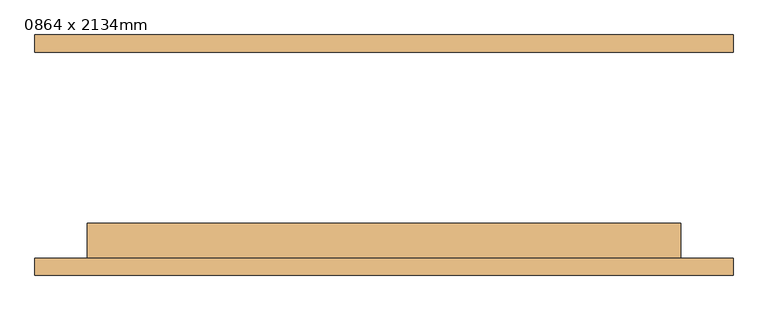
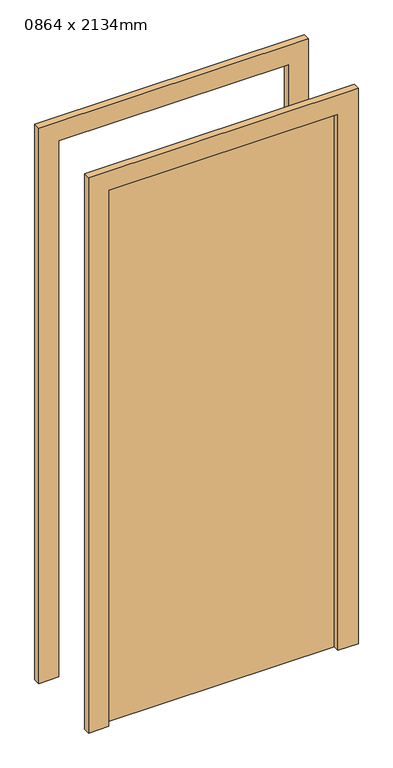
"""IFC4 building model written with IfcOpenShell, lengths in millimetres: door geometry, M_Folha única : 0864 x 2134mm."""

from ifc_helpers import new_model, si_unit, frame, origin, origin_with_axes, place, context, project, spatial, polyline, outline, extrude, source, transform, mapped, element, save


def door_0864_x_2134mm_1beed8f0(model_context):
    return source(origin(), model_context, "Body", "SweptSolid", [
        extrude(outline(polyline([(2210.0, -508.0), (0.0, -508.0), (0.0, -432.0), (2134.0, -432.0), (2134.0, 432.0), (0.0, 432.0), (0.0, 508.0), (2210.0, 508.0), (2210.0, -508.0)])), frame((0.0, -175.0, 0.0), z_axis=(0.0, 1.0, 0.0), x_axis=(0.0, 0.0, 1.0)), (0.0, 0.0, 1.0), 25.0),
        extrude(outline(polyline([(2210.0, 508.0), (2210.0, -508.0), (0.0, -508.0), (0.0, -432.0), (2134.0, -432.0), (2134.0, 432.0), (0.0, 432.0), (0.0, 508.0), (2210.0, 508.0)])), frame((0.0, 150.0, 0.0), z_axis=(0.0, 1.0, 0.0), x_axis=(0.0, 0.0, 1.0)), (0.0, 0.0, 1.0), 25.0),
        extrude(outline(polyline([(432.0, -99.0), (432.0, -150.0), (-432.0, -150.0), (-432.0, -99.0), (432.0, -99.0)])), origin_with_axes(), (0.0, 0.0, 1.0), 2134.0),
    ])


if __name__ == "__main__":
    model = new_model("IFC4")
    model_context = context("Model", 3, world=origin())
    ifc_project = project(units=[si_unit("LENGTHUNIT", "METRE", prefix="MILLI")], contexts=[model_context])
    site = spatial("IfcSite", under=ifc_project)
    building = spatial("IfcBuilding", under=site)
    placement = place(None, origin())
    door_0864_x_2134mm_shape = door_0864_x_2134mm_1beed8f0(model_context)
    element("IfcDoor", 1, ObjectType="M_Folha única : 0864 x 2134mm", at=placement, inside=building, context=model_context, shape_type="MappedRepresentation", body=[
        mapped(door_0864_x_2134mm_shape, transform((0.0, 0.0, 0.0), x_axis=(1.0, 0.0, 0.0), y_axis=(0.0, 1.0, 0.0), z_axis=(0.0, 0.0, 1.0))),
    ])
    save(model, "model.ifc")

# Revit data of these elements
# Project information
#   Opção de desenho = "Modelo principal"
#   Data de emissão do projeto = "Data de emissão"
#   Status do projeto = "Status do projeto"
#   Nome do cliente = "Proprietário"
#   Endereço do projeto = "Insira aqui o endereço"
#   Nome do projeto = "Nome do projeto"
#   Número do projeto = "0001"
# Type "M_Folha única : 0864 x 2134mm"
#   Type Mark = "22"
#   Construction Type Id = "MDOOR"
#   Analytic Construction = "Metal"
#   Thickness = 0.051 m
#   Thermal Resistance (R) = 0.270117 (m²·K)/W
#   Heat Transfer Coefficient (U) = 3.7021 W/(m²·K)
#   Height = 2.134 m
#   Projeção da apara externa = 0.025 m
#   Projeção da apara interna = 0.025 m
#   Largura da apara = 0.076 m
#   Width = 0.864 m
#   Define Thermal Properties by = 1
#   Define Thermal Properties by = 1
#   Material da porta = Porta - Painel
#   Material da moldura = Porta - Batente
#   Visual Light Transmittance = 0
#   Solar Heat Gain Coefficient = 0
#   Function = (empty or 0)
#   Wall Closure = (empty or 0)
# Element 1 (IfcDoor, "M_Folha única : 0864 x 2134mm")
#   Materials on its faces: "Porta - Batente", "Porta - Painel"
# Materials
#   "Porta - Painel": class "Madeira", colour RGB 210 159 95, transparency 0, Cost = 0
#   "Porta - Batente": class "Diversos", colour RGB 118 70 51, transparency 0, Cost = 0
